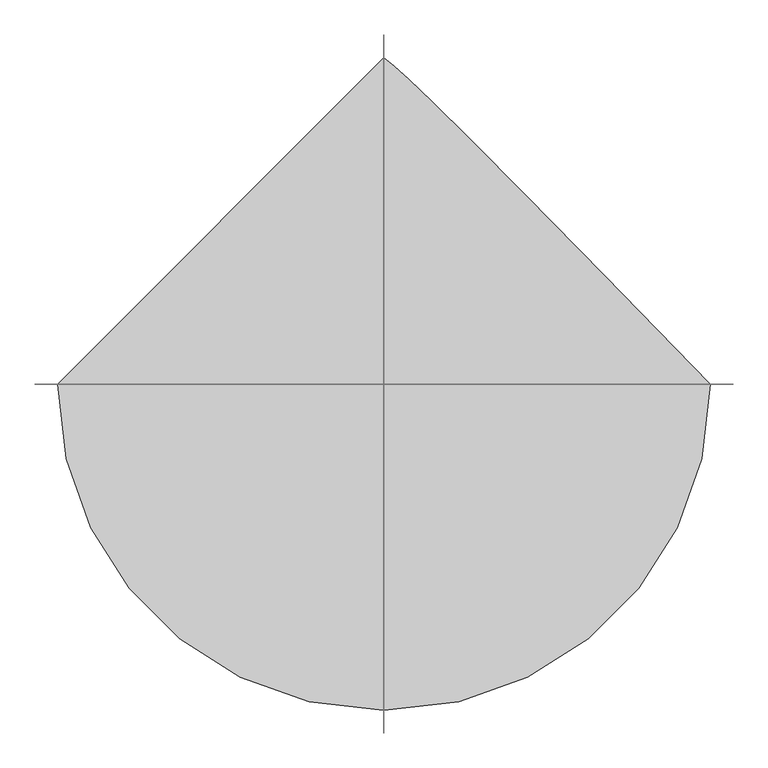
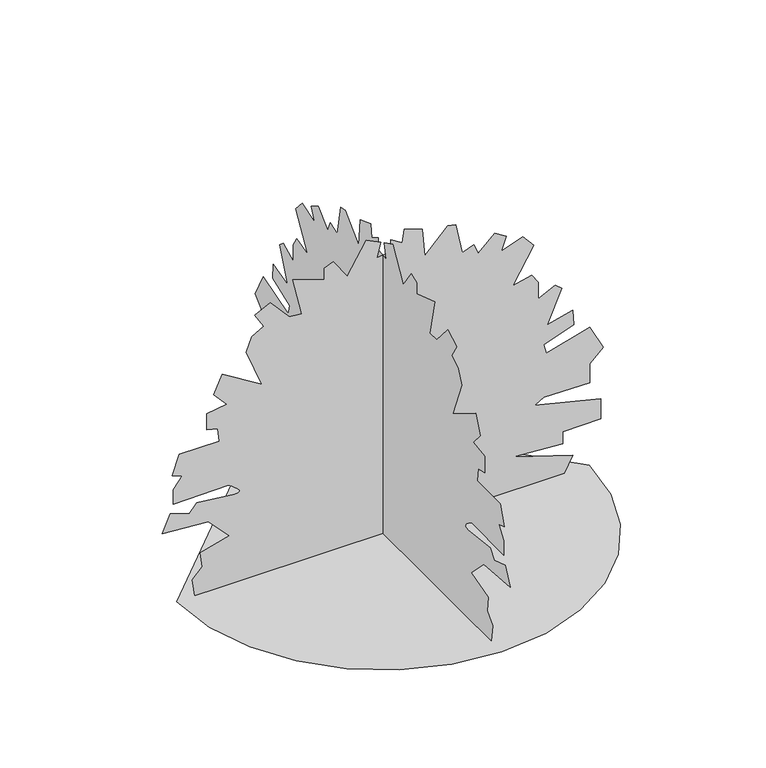
"""IFC4 building model written with IfcOpenShell, lengths in millimetres: proxy geometry, privet 26761 : privet 26761."""

from ifc_helpers import new_model, si_unit, origin, place, context, project, spatial, triangles, source, transform, mapped, element, save


def entourage_76426c84(model_context):
    return source(origin(), model_context, "Body", "Tessellation", [
        triangles([(-629.6484856, 0.0, 4.95e-05), (-613.003862, -144.2738427, 4.95e-05), (-565.5947282, -276.766137, 4.95e-05), (-491.2235046, -393.6824018, 4.95e-05), (-393.6824018, -491.2235046, 4.95e-05), (-276.766137, -565.5947282, 4.95e-05), (-144.2738427, -613.003862, 4.95e-05), (2.75e-05, -629.6484856, 4.95e-05), (144.2738427, -613.003862, 4.95e-05), (276.766137, -565.5947282, 4.95e-05), (393.6824018, -491.2235046, 4.95e-05), (491.2235046, -393.6824018, 4.95e-05), (565.5947282, -276.766137, 4.95e-05), (613.003862, -144.2738427, 4.95e-05), (629.6484856, 5.5e-05, 4.95e-05), (425.0259828, 209.8919668, 4.95e-05), (273.329519, 364.4266657, 4.95e-05), (165.7386299, 472.8288062, 4.95e-05), (93.4306343, 544.3247692, 4.95e-05), (47.5853949, 588.1448779, 4.95e-05), (19.3822403, 613.5093544, 4.95e-05), (-8.26e-05, 629.6484856, 4.95e-05), (-2.3e-06, -573.7887774, 0.0), (-2.3e-06, -582.0844193, 55.3049682), (-2.3e-06, -551.6679256, 85.7227472), (-2.3e-06, -557.1974936, 132.7320781), (0.0, -468.7089269, 157.747784), (0.0, -532.310568, 224.1137004), (0.0, -673.33906, 235.174635), (0.0, -648.4495909, 290.4795987), (0.0, -590.3800612, 271.1222591), (0.0, -568.2592094, 298.7752406), (0.0, -452.1176431, 284.9500125), (0.0, -441.363285, 285.9964966), (0.0, -436.849716, 288.9327454), (0.0, -437.5355026, 293.4387022), (0.0, -442.379284, 299.2019587), (0.0, -450.3447135, 305.9101067), (0.0, -460.3904303, 313.2456327), (0.0, -471.4750008, 320.898654), (0.0, -640.153949, 318.1325801), (0.0, -640.153949, 365.1403939), (0.0, -612.5034565, 401.0890354), (0.0, -642.9199865, 412.1507512), (0.0, -620.7990984, 472.9863184), (0.0, -499.1280004, 472.9863184), (0.0, -504.6575684, 514.4645279), (0.0, -537.840136, 522.7601698), (0.0, -537.840136, 575.3000951), (0.0, -477.0045688, 583.595737), (0.0, -515.7192842, 627.8400204), (0.0, -490.8323585, 685.9095137), (0.0, -369.1612241, 611.2487366), (0.0, -416.1690016, 730.1537607), (0.0, -399.5777178, 774.3980804), (0.0, -363.6291126, 796.521512), (0.0, -391.2820759, 840.7632156), (0.0, -344.2742984, 865.6526848), (0.0, -286.2022435, 799.2850061), (0.0, -247.4898354, 796.521512), (0.0, -275.1430711, 915.4265362), (0.0, -178.3586263, 882.2439686), (0.0, -178.3586263, 918.190103), (0.0, -150.7061354, 929.2517824), (0.0, -109.2271628, 868.4161789), (0.0, -51.1571472, 965.2003876), (0.0, -6.9130699, 943.0795721), (0.0, -17.9741141, 896.0692148), (0.0, 23.5046359, 901.5988192), (0.0, 23.5046359, 940.3134619), (0.0, 59.4527891, 918.190103), (0.0, 64.9833881, 959.6708559), (0.0, 120.2883518, 940.3134619), (0.0, 128.5842571, 851.8248951), (0.0, 197.7154571, 923.7221781), (0.0, 222.6026553, 918.190103), (0.0, 241.9594862, 821.4084377), (0.0, 277.9066016, 835.2336113), (0.0, 291.7343731, 802.0510437), (0.0, 341.5082245, 849.0588575), (0.0, 377.456866, 826.9379694), (0.0, 360.8655822, 785.4597599), (0.0, 427.2307174, 807.580648), (0.0, 460.413285, 768.8684761), (0.0, 396.8142237, 661.022588), (0.0, 454.883717, 674.8503777), (0.0, 474.2410747, 644.4313042), (0.0, 474.2410747, 591.8913789), (0.0, 526.7809999, 616.7782682), (0.0, 546.1357779, 600.1870208), (0.0, 501.8915308, 497.8732441), (0.0, 579.3183818, 517.2305655), (0.0, 582.0844193, 470.2202445), (0.0, 490.8323585, 437.0376769), (0.0, 499.1280004, 406.6211469), (0.0, 631.8583071, 445.3333188), (0.0, 673.33906, 365.1403939), (0.0, 631.8583071, 326.428222), (0.0, 631.8583071, 265.592673), (0.0, 490.8323585, 268.3587287), (0.0, 463.1793589, 251.7661732), (0.0, 665.0434181, 201.9918131), (0.0, 665.0434181, 138.3909441), (0.0, 548.9018517, 135.6256423), (0.0, 548.9018517, 96.9122169), (0.0, 399.5777178, 107.9731605), (0.0, 579.3183818, 49.9031495), (0.0, 554.4314198, 0.1285451), (-573.7887774, 9.96e-05, 4.86e-05), (-582.0844193, 9.63e-05, 55.3049682), (-551.6679256, 9.44e-05, 85.7227472), (-557.1974936, 9.16e-05, 132.7320781), (-468.7089269, 8.79e-05, 157.747784), (-532.310568, 8.39e-05, 224.1137004), (-673.33906, 8.33e-05, 235.174635), (-648.4495909, 8e-05, 290.4795987), (-590.3800612, 8.11e-05, 271.1222591), (-568.2592094, 7.95e-05, 298.7752406), (-452.1176431, 8.03e-05, 284.9500125), (-441.363285, 8.02e-05, 285.9964966), (-436.849716, 8.01e-05, 288.9327454), (-437.5355026, 7.98e-05, 293.4387022), (-442.379284, 7.95e-05, 299.2019587), (-450.3447135, 7.91e-05, 305.9101067), (-460.3904303, 7.86e-05, 313.2456327), (-471.4750008, 7.82e-05, 320.898654), (-640.153949, 7.83e-05, 318.1325801), (-640.153949, 7.55e-05, 365.1403939), (-612.5034565, 7.34e-05, 401.0890354), (-642.9199865, 7.27e-05, 412.1507512), (-620.7990984, 6.91e-05, 472.9863184), (-499.1280004, 6.91e-05, 472.9863184), (-504.6575684, 6.66e-05, 514.4645279), (-537.840136, 6.61e-05, 522.7601698), (-537.840136, 6.3e-05, 575.3000951), (-477.0045688, 6.25e-05, 583.595737), (-515.7192842, 5.99e-05, 627.8400204), (-490.8323585, 5.64e-05, 685.9095137), (-369.1612241, 6.09e-05, 611.2487366), (-416.1690016, 5.38e-05, 730.1537607), (-399.5777178, 5.11e-05, 774.3980804), (-363.6291126, 4.98e-05, 796.521512), (-391.2820759, 4.72e-05, 840.7632156), (-344.2742984, 4.57e-05, 865.6526848), (-286.2022435, 4.96e-05, 799.2850061), (-247.4898354, 4.98e-05, 796.521512), (-275.1430711, 4.27e-05, 915.4265362), (-178.3586263, 4.47e-05, 882.2439686), (-178.3586263, 4.26e-05, 918.190103), (-150.7061354, 4.19e-05, 929.2517824), (-109.2274081, 4.55e-05, 868.4161789), (-51.1571472, 3.98e-05, 965.2003876), (-6.9131466, 4.11e-05, 943.0795721), (-17.9741902, 4.39e-05, 896.0692148), (23.5045859, 4.35e-05, 901.5988192), (23.5045859, 4.12e-05, 940.3134619), (59.4527891, 4.26e-05, 918.190103), (64.9833881, 4.01e-05, 959.6708559), (120.2883518, 4.12e-05, 940.3134619), (128.5840028, 4.65e-05, 851.8248951), (197.7152028, 4.22e-05, 923.7221781), (222.6026553, 4.26e-05, 918.190103), (241.9592318, 4.83e-05, 821.4084377), (277.9066016, 4.75e-05, 835.2336113), (291.7343731, 4.95e-05, 802.0510437), (341.5082245, 4.67e-05, 849.0588575), (377.456866, 4.8e-05, 826.9379694), (360.8655822, 5.05e-05, 785.4597599), (427.2307174, 4.92e-05, 807.580648), (460.413285, 5.15e-05, 768.8684761), (396.8142237, 5.79e-05, 661.022588), (454.883717, 5.71e-05, 674.8503777), (474.2410747, 5.89e-05, 644.4313042), (474.2410747, 6.2e-05, 591.8913789), (526.7809999, 6.05e-05, 616.7782682), (546.1357779, 6.15e-05, 600.1870208), (501.8915308, 6.76e-05, 497.8732441), (579.3183818, 6.65e-05, 517.2305655), (582.0844193, 6.93e-05, 470.2202445), (490.8323585, 7.12e-05, 437.0376769), (499.1280004, 7.31e-05, 406.6211469), (631.8583071, 7.07e-05, 445.3333188), (673.33906, 7.55e-05, 365.1403939), (631.8583071, 7.78e-05, 326.428222), (631.8583071, 8.15e-05, 265.592673), (490.8323585, 8.13e-05, 268.3587287), (463.1793589, 8.23e-05, 251.7661732), (665.0434181, 8.52e-05, 201.9918131), (665.0434181, 8.9e-05, 138.3909441), (548.9018517, 8.92e-05, 135.6258967), (548.9018517, 9.15e-05, 96.9122169), (399.5777178, 9.09e-05, 107.9734149), (579.3183818, 9.43e-05, 49.9031495), (554.4314198, 9.73e-05, 0.1285937)], [[21, 22, 1], [20, 21, 1], [19, 20, 1], [18, 19, 1], [17, 18, 1], [17, 1, 2], [17, 2, 3], [17, 3, 4], [16, 17, 4], [16, 4, 5], [16, 5, 6], [16, 6, 7], [16, 7, 8], [16, 8, 9], [16, 9, 10], [16, 10, 11], [16, 11, 12], [15, 16, 12], [14, 15, 12], [13, 14, 12], [60, 61, 62], [69, 70, 71], [28, 29, 30], [28, 30, 31], [71, 72, 73], [71, 73, 74], [91, 92, 93], [91, 93, 94], [106, 107, 108], [106, 108, 23], [51, 52, 53], [50, 51, 53], [104, 105, 106], [56, 57, 58], [56, 58, 59], [98, 99, 100], [40, 41, 42], [40, 42, 43], [43, 44, 45], [43, 45, 46], [40, 43, 46], [28, 31, 32], [102, 103, 104], [101, 102, 104], [101, 104, 106], [77, 78, 79], [106, 23, 24], [106, 24, 25], [65, 66, 67], [65, 67, 68], [106, 25, 26], [106, 26, 27], [48, 49, 50], [47, 48, 50], [80, 81, 82], [79, 80, 82], [95, 96, 97], [95, 97, 98], [95, 98, 100], [63, 64, 65], [62, 63, 65], [89, 90, 91], [88, 89, 91], [27, 28, 32], [27, 32, 33], [106, 27, 33], [106, 33, 34], [106, 34, 35], [101, 106, 35], [101, 35, 36], [83, 84, 85], [82, 83, 85], [85, 86, 87], [85, 87, 88], [69, 71, 74], [75, 76, 77], [74, 75, 77], [60, 62, 65], [79, 82, 85], [95, 100, 101], [95, 101, 36], [94, 95, 36], [91, 94, 36], [88, 91, 36], [85, 88, 36], [79, 85, 36], [77, 79, 36], [74, 77, 36], [69, 74, 36], [68, 69, 36], [65, 68, 36], [60, 65, 36], [60, 36, 37], [60, 37, 38], [59, 60, 38], [59, 38, 39], [59, 39, 40], [47, 50, 53], [46, 47, 53], [40, 46, 53], [59, 40, 53], [59, 53, 54], [56, 59, 54], [56, 54, 55], [146, 147, 148], [155, 156, 157], [114, 115, 116], [114, 116, 117], [157, 158, 159], [157, 159, 160], [177, 178, 179], [177, 179, 180], [192, 193, 194], [192, 194, 109], [137, 138, 139], [136, 137, 139], [190, 191, 192], [142, 143, 144], [142, 144, 145], [184, 185, 186], [126, 127, 128], [126, 128, 129], [129, 130, 131], [129, 131, 132], [126, 129, 132], [114, 117, 118], [188, 189, 190], [187, 188, 190], [187, 190, 192], [163, 164, 165], [192, 109, 110], [192, 110, 111], [151, 152, 153], [151, 153, 154], [192, 111, 112], [192, 112, 113], [134, 135, 136], [133, 134, 136], [166, 167, 168], [165, 166, 168], [181, 182, 183], [181, 183, 184], [181, 184, 186], [149, 150, 151], [148, 149, 151], [175, 176, 177], [174, 175, 177], [113, 114, 118], [113, 118, 119], [192, 113, 119], [192, 119, 120], [192, 120, 121], [187, 192, 121], [187, 121, 122], [169, 170, 171], [168, 169, 171], [171, 172, 173], [171, 173, 174], [155, 157, 160], [161, 162, 163], [160, 161, 163], [146, 148, 151], [165, 168, 171], [181, 186, 187], [181, 187, 122], [180, 181, 122], [177, 180, 122], [174, 177, 122], [171, 174, 122], [165, 171, 122], [163, 165, 122], [160, 163, 122], [155, 160, 122], [154, 155, 122], [151, 154, 122], [146, 151, 122], [146, 122, 123], [146, 123, 124], [145, 146, 124], [145, 124, 125], [145, 125, 126], [133, 136, 139], [132, 133, 139], [126, 132, 139], [145, 126, 139], [145, 139, 140], [142, 145, 140], [142, 140, 141]], closed=False),
    ])


if __name__ == "__main__":
    model = new_model("IFC4")
    model_context = context("Model", 3, world=origin())
    ifc_project = project(units=[si_unit("LENGTHUNIT", "METRE", prefix="MILLI")], contexts=[model_context])
    site = spatial("IfcSite", under=ifc_project)
    building = spatial("IfcBuilding", under=site)
    placement = place(None, origin())
    entourage_shape = entourage_76426c84(model_context)
    element("IfcBuildingElementProxy", 1, Name="privet 26761 : privet 26761", ObjectType="privet 26761 : privet 26761", at=placement, inside=building, context=model_context, shape_type="MappedRepresentation", body=[
        mapped(entourage_shape, transform((0.0, 0.0, 0.0), x_axis=(1.0, 0.0, 0.0), y_axis=(0.0, 1.0, 0.0), z_axis=(0.0, 0.0, 1.0))),
    ])
    save(model, "model.ifc")

# Revit data of these elements
# Type "privet 26761 : privet 26761"
#   built-in parameter 1005195 = "RPC-16-FXGX-NJPX-PH0L-8000-ST1L-LVER-AU"
#   Height = 0
